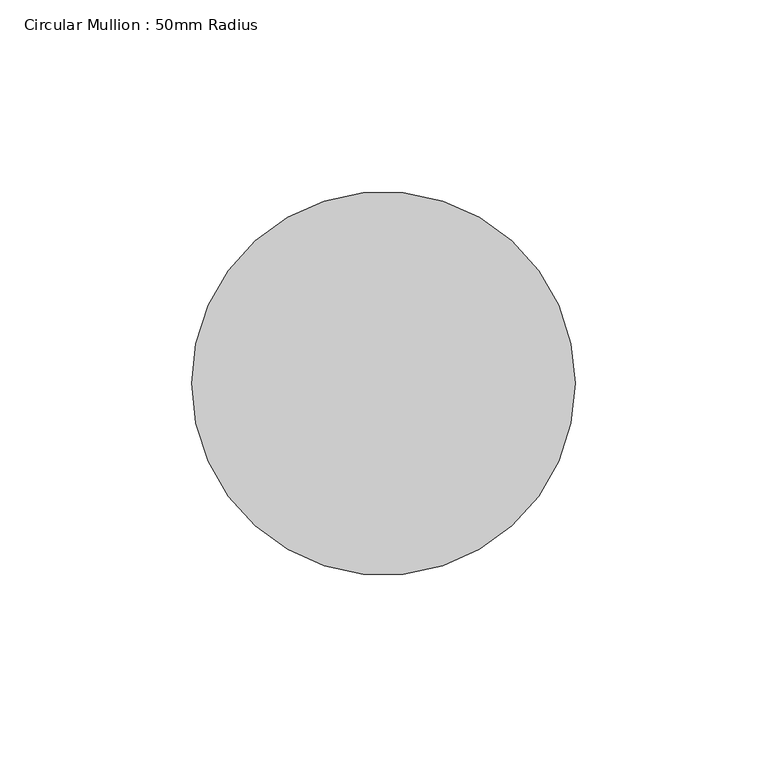
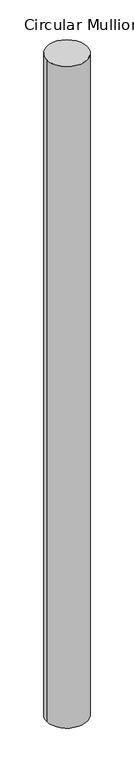
"""IFC4 building model written with IfcOpenShell, lengths in millimetres: member geometry, Circular Mullion : 50mm Radius."""

from ifc_helpers import new_model, si_unit, point, frame, origin, origin_2d, place, context, project, spatial, circle_curve, trimmed, segment, composite_curve, outline, extrude, source, transform, mapped, element, save


def circular_mullion_50mm_radius_b18170ad(model_context):
    return source(origin(), model_context, "Body", "SweptSolid", [
        extrude(outline(composite_curve([segment(trimmed(circle_curve(origin_2d(), 50.0), [point((50.0, 0.0))], [point((-50.0, 0.0))], False, "CARTESIAN"), True, "CONTINUOUS"), segment(trimmed(circle_curve(origin_2d(), 50.0), [point((-50.0, 0.0))], [point((50.0, 0.0))], False, "CARTESIAN"), True, "CONTINUOUS")], self_intersect=False)), frame((0.0, 0.0, -1727.2933627), z_axis=(0.0, 0.0, 1.0), x_axis=(1.0, 0.0, 0.0)), (0.0, 0.0, 1.0), 1727.2933627),
    ])


if __name__ == "__main__":
    model = new_model("IFC4")
    model_context = context("Model", 3, world=origin())
    ifc_project = project(units=[si_unit("LENGTHUNIT", "METRE", prefix="MILLI")], contexts=[model_context])
    site = spatial("IfcSite", under=ifc_project)
    building = spatial("IfcBuilding", under=site)
    placement = place(None, origin())
    circular_mullion_50mm_radius_shape = circular_mullion_50mm_radius_b18170ad(model_context)
    element("IfcMember", 1, ObjectType="Circular Mullion : 50mm Radius", at=placement, inside=building, context=model_context, shape_type="MappedRepresentation", body=[
        mapped(circular_mullion_50mm_radius_shape, transform((0.0, 0.0, 0.0), x_axis=(1.0, 0.0, 0.0), y_axis=(0.0, 1.0, 0.0), z_axis=(0.0, 0.0, 1.0))),
    ])
    save(model, "model.ifc")

# Revit data of these elements
# Type "Circular Mullion : 50mm Radius"
#   built-in parameter 1007350 = 0.164042 (stored number, unit not read)
# Element 1 (IfcMember, "Circular Mullion : 50mm Radius")
#   Materials on its faces: "Aluminium"
# Materials
#   "Aluminium": class "Metal", colour RGB 247 247 247, transparency 0, Description = "Aluminium 6061", Cost = 0
